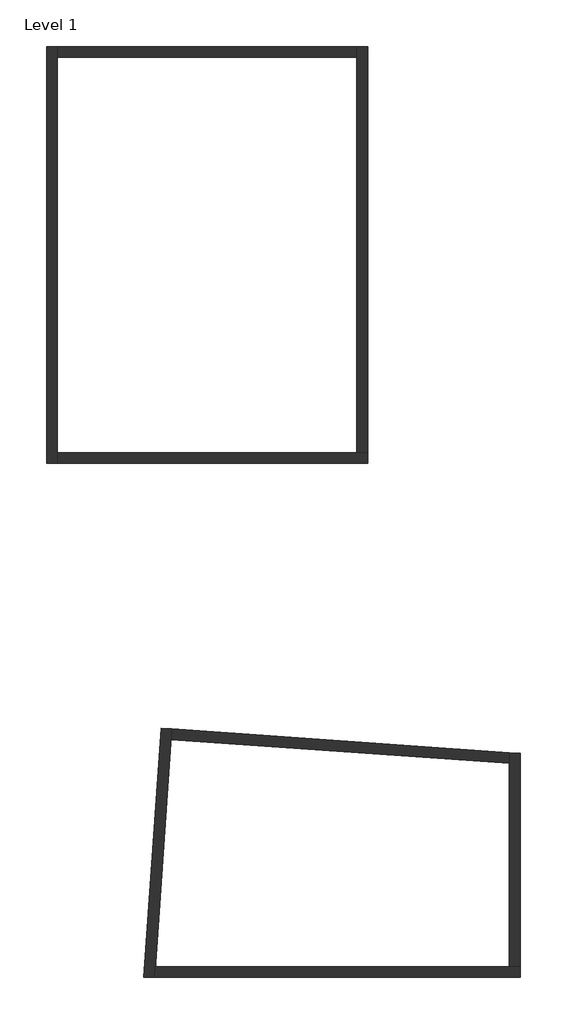
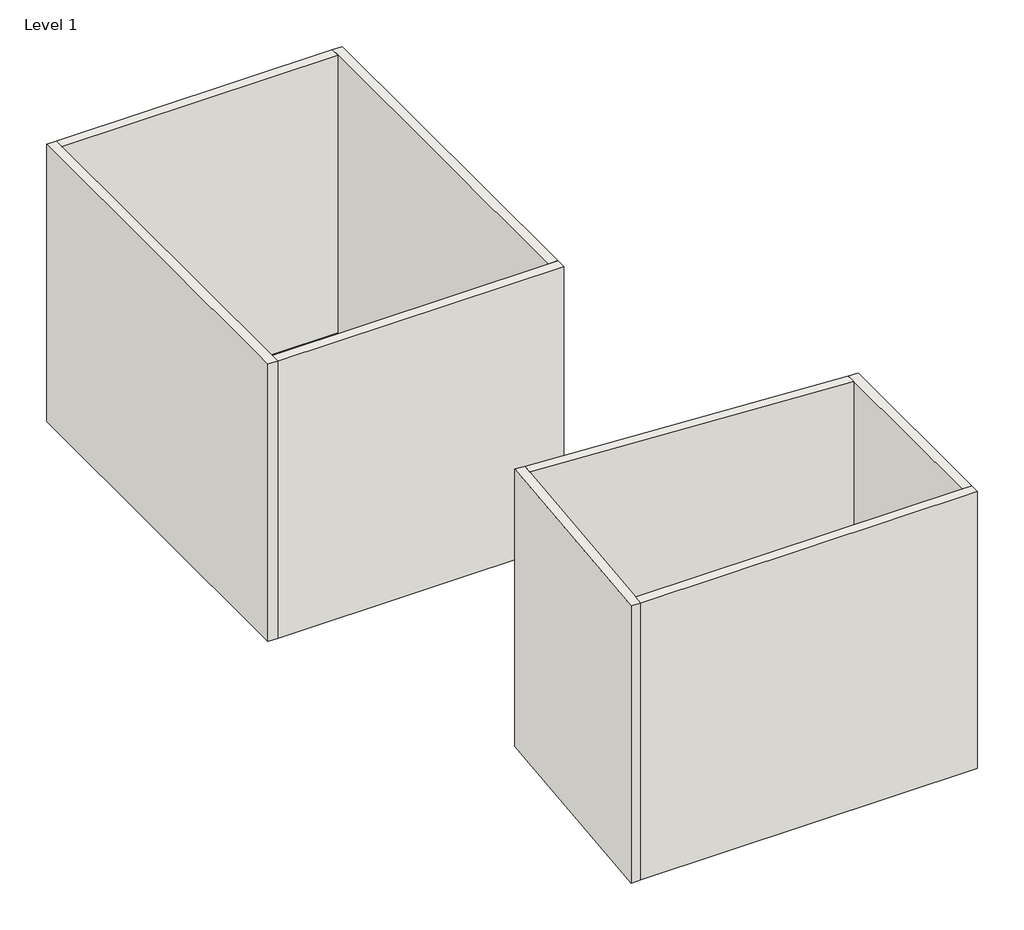
# One storey: 8 walls.
"""IFC4 building model written with IfcOpenShell, lengths in millimetres."""

from ifc_helpers import new_model, si_unit, origin, origin_with_axes, place, context, project, spatial, polyline, outline, extrude, faceted_brep, element, save

model = new_model("IFC4")

# Units and contexts
model_context = context("Model", 3, world=origin())
ifc_project = project(units=[si_unit("LENGTHUNIT", "METRE", prefix="MILLI")], contexts=[model_context])

# Site, building, storey
site = spatial("IfcSite", under=ifc_project)
building = spatial("IfcBuilding", under=site)
storey = spatial("IfcBuildingStorey", under=building, Name="Level 1", Elevation=0.0)

# Walls
placement = place(None, origin())
element("IfcWall", 1, ObjectType="Generic - 8\"", at=placement, inside=storey, context=model_context, shape_type="Brep", body=[
    faceted_brep([(-16217.1430934, 9060.6311633, 0.0), (-16217.1430934, 1085.0311633, 0.0), (-16217.1430934, 1085.0311633, 6096.0), (-16217.1430934, 9060.6311633, 6096.0), (-16013.9430934, 9060.6311633, 0.0), (-16013.9430934, 9060.6311633, 6096.0), (-16013.9430934, 8857.4311633, 6096.0), (-16013.9430934, 1288.2311633, 6096.0), (-16013.9430934, 1085.0311633, 6096.0), (-16013.9430934, 1085.0311633, 0.0), (-16013.9430934, 1288.2311633, 0.0), (-16013.9430934, 8857.4311633, 0.0)], [[[0, 1, 2, 3]], [[4, 5, 6, 7, 8, 9, 10, 11]], [[1, 0, 4, 11, 10, 9]], [[3, 2, 8, 7, 6, 5]], [[2, 1, 9, 8]], [[0, 3, 5, 4]]]),
])
element("IfcWall", 2, ObjectType="Generic - 8\"", at=placement, inside=storey, context=model_context, shape_type="Brep", body=[
    faceted_brep([(-16013.9430934, 1085.0311633, 0.0), (-10070.3430934, 1085.0311633, 0.0), (-10070.3430934, 1085.0311633, 6096.0), (-16013.9430934, 1085.0311633, 6096.0), (-16013.9430934, 1288.2311633, 0.0), (-16013.9430934, 1288.2311633, 6096.0), (-10273.5430934, 1288.2311633, 6096.0), (-10070.3430934, 1288.2311633, 6096.0), (-10070.3430934, 1288.2311633, 0.0), (-10273.5430934, 1288.2311633, 0.0)], [[[0, 1, 2, 3]], [[4, 5, 6, 7, 8, 9]], [[1, 0, 4, 9, 8]], [[3, 2, 7, 6, 5]], [[0, 3, 5, 4]], [[2, 1, 8, 7]]]),
])
element("IfcWall", 3, ObjectType="Generic - 8\"", at=placement, inside=storey, context=model_context, shape_type="Brep", body=[
    faceted_brep([(-10070.3430934, 1288.2311633, 0.0), (-10070.3430934, 9060.6311633, 0.0), (-10070.3430934, 9060.6311633, 6096.0), (-10070.3430934, 1288.2311633, 6096.0), (-10273.5430934, 1288.2311633, 0.0), (-10273.5430934, 1288.2311633, 6096.0), (-10273.5430934, 8857.4311633, 6096.0), (-10273.5430934, 9060.6311633, 6096.0), (-10273.5430934, 9060.6311633, 0.0), (-10273.5430934, 8857.4311633, 0.0)], [[[0, 1, 2, 3]], [[4, 5, 6, 7, 8, 9]], [[1, 0, 4, 9, 8]], [[3, 2, 7, 6, 5]], [[0, 3, 5, 4]], [[2, 1, 8, 7]]]),
])
element("IfcWall", 4, ObjectType="Generic - 8\"", at=placement, inside=storey, context=model_context, shape_type="SweptSolid", body=[
    extrude(outline(polyline([(-16013.9430934, 9060.6311633), (-10273.5430934, 9060.6311633), (-10273.5430934, 8857.4311633), (-16013.9430934, 8857.4311633), (-16013.9430934, 9060.6311633)])), origin_with_axes(), (0.0, 0.0, 1.0), 6096.0),
])
element("IfcWall", 5, ObjectType="Generic - 8\"", at=placement, inside=storey, context=model_context, shape_type="Brep", body=[
    faceted_brep([(-14018.0232115, -3991.3589408, 0.0), (-14351.6372206, -8762.2615438, 0.0), (-14351.6372206, -8762.2615438, 6096.0), (-14018.0232115, -3991.3589408, 6096.0), (-13815.3181965, -4005.5334563, 0.0), (-13815.3181965, -4005.5334563, 6096.0), (-13829.492712, -4208.2384713, 6096.0), (-14133.7318988, -8559.0615438, 6096.0), (-14147.9410269, -8762.2615438, 6096.0), (-14147.9410269, -8762.2615438, 0.0), (-14133.7318988, -8559.0615438, 0.0), (-13829.492712, -4208.2384713, 0.0)], [[[0, 1, 2, 3]], [[4, 5, 6, 7, 8, 9, 10, 11]], [[1, 0, 4, 11, 10, 9]], [[3, 2, 8, 7, 6, 5]], [[2, 1, 9, 8]], [[0, 3, 5, 4]]]),
])
element("IfcWall", 6, ObjectType="Generic - 8\"", at=placement, inside=storey, context=model_context, shape_type="Brep", body=[
    faceted_brep([(-14147.9410269, -8762.2615438, 0.0), (-7150.6008385, -8762.2615438, 0.0), (-7150.6008385, -8762.2615438, 6096.0), (-14147.9410269, -8762.2615438, 6096.0), (-14133.7318988, -8559.0615438, 0.0), (-14133.7318988, -8559.0615438, 6096.0), (-7353.8008385, -8559.0615438, 6096.0), (-7150.6008385, -8559.0615438, 6096.0), (-7150.6008385, -8559.0615438, 0.0), (-7353.8008385, -8559.0615438, 0.0)], [[[0, 1, 2, 3]], [[4, 5, 6, 7, 8, 9]], [[1, 0, 4, 9, 8]], [[3, 2, 7, 6, 5]], [[0, 3, 5, 4]], [[2, 1, 8, 7]]]),
])
element("IfcWall", 7, ObjectType="Generic - 8\"", at=placement, inside=storey, context=model_context, shape_type="Brep", body=[
    faceted_brep([(-7150.6008385, -8559.0615438, 0.0), (-7150.6008385, -4471.5758936, 0.0), (-7150.6008385, -4471.5758936, 6096.0), (-7150.6008385, -8559.0615438, 6096.0), (-7353.8008385, -8559.0615438, 0.0), (-7353.8008385, -8559.0615438, 6096.0), (-7353.8008385, -4661.0629591, 6096.0), (-7353.8008385, -4457.3667654, 6096.0), (-7353.8008385, -4457.3667654, 0.0), (-7353.8008385, -4661.0629591, 0.0)], [[[0, 1, 2, 3]], [[4, 5, 6, 7, 8, 9]], [[1, 0, 4, 9, 8]], [[3, 2, 7, 6, 5]], [[0, 3, 5, 4]], [[2, 1, 8, 7]]]),
])
element("IfcWall", 8, ObjectType="Generic - 8\"", at=placement, inside=storey, context=model_context, shape_type="SweptSolid", body=[
    extrude(outline(polyline([(-13815.3181965, -4005.5334563), (-7353.8008385, -4457.3667654), (-7353.8008385, -4661.0629591), (-13829.492712, -4208.2384713), (-13815.3181965, -4005.5334563)])), origin_with_axes(), (0.0, 0.0, 1.0), 6096.0),
])

save(model, "model.ifc")

# Revit data of these elements
# Project information
#   Project Issue Date = "Issue Date"
#   Project Status = "Project Status"
#   Client Name = "Owner"
#   Project Address = "Enter address here"
#   Project Name = "Project Name"
#   Project Number = "Project Number"
# Type "Generic - 8\""
#   Assembly Code = "B2010"
#   Layers, outside or top first: 0' - 8" no material (function 1)
# Elements 1, 2, 3, 4, 5, 6, 7, 8 (IfcWall, "Generic - 8\"")
#   Top Offset = 0' - 0"
#   Base Offset = 0' - 0"
#   Unconnected Height = 20' - 0"
#   wall height = 20' - 0"
#   Phase Created = New Construction
#   Base Constraint = Level 1
#   Materials on its faces: "Default Wall"
# Materials
#   "Default Wall": class "Miscellaneous", colour RGB 128 128 128, transparency 0, Cost = 0
# Room at (-10876.127, -6654.883) mm, phase "New Construction", upper level "Level 1", upper offset 10' - 0", lower offset 0' - 0"
#   Number = "2"
#   Name = "Room"
# Room at (-12397.129, 5692.09) mm, phase "New Construction", upper level "Level 1", upper offset 10' - 0", lower offset 0' - 0"
#   Number = "1"
#   Name = "string stringssssss stringstringstring stringstringstring string string sssssssssssss ssssss"
